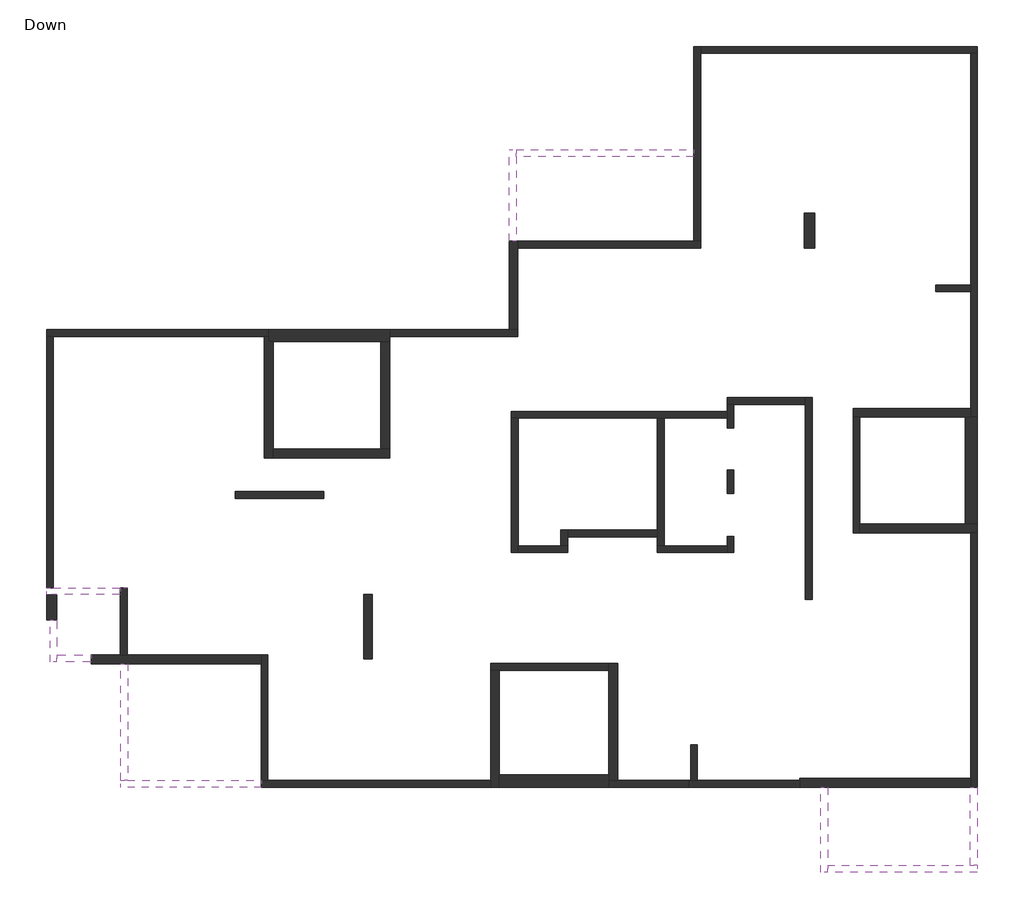
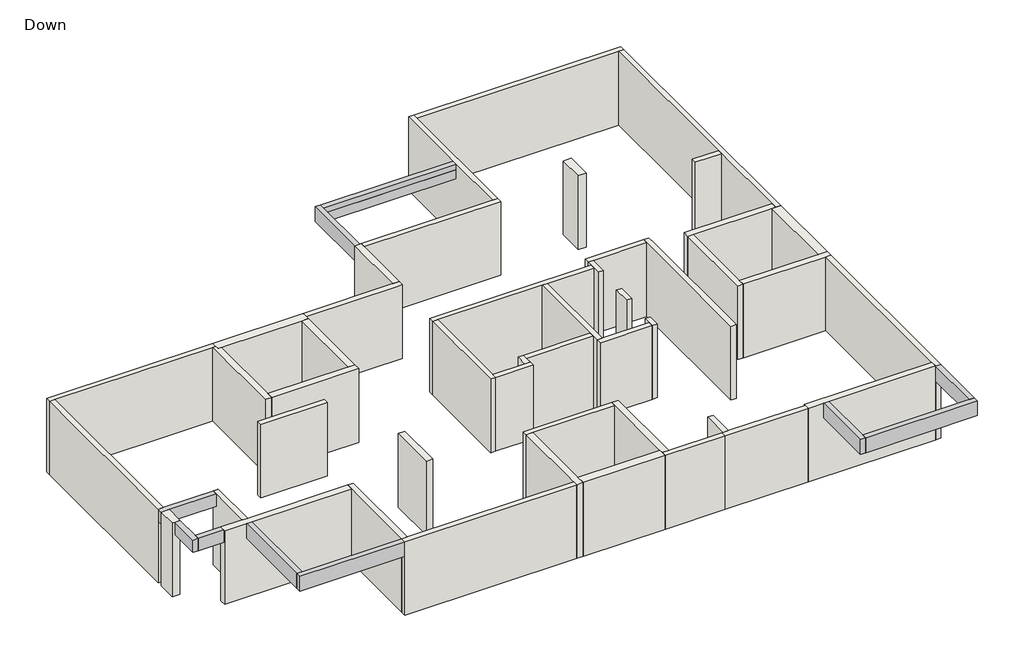
# One storey: 46 walls, 10 beams.
"""IFC4 building model written with IfcOpenShell, lengths in millimetres."""

from ifc_helpers import new_model, si_unit, frame, origin, place, context, project, spatial, polyline, outline, extrude, faceted_brep, element, save

model = new_model("IFC4")

# Units and contexts
model_context = context("Model", 3, world=origin())
ifc_project = project(units=[si_unit("LENGTHUNIT", "METRE", prefix="MILLI")], contexts=[model_context])

# Site, building, storey
site = spatial("IfcSite", under=ifc_project)
building = spatial("IfcBuilding", under=site)
storey = spatial("IfcBuildingStorey", under=building, Name="Down", Elevation=0.0)

# Beams
placement = place(None, origin())
element("IfcBeam", 1, ObjectType="Concrete Rectengular Beam : 20/50", at=placement, inside=storey, context=model_context, shape_type="Brep", body=[
    faceted_brep([(-17264.6329455, 698.5534768, 3000.0), (-17264.6329455, 502.021863, 3000.0), (-16964.6329455, 502.021863, 3000.0), (-15146.7835264, 502.021863, 3000.0), (-15146.7835264, 701.4062462, 3000.0), (-14946.7835264, 701.4062462, 3000.0), (-14946.7835264, 702.021863, 3000.0), (-17064.6329455, 702.021863, 3000.0), (-17064.6329455, 698.5534768, 3000.0), (-17264.6329455, 502.021863, 2500.0), (-15146.7835264, 502.021863, 2500.0), (-15146.7835264, 502.021863, 2770.0), (-17264.6329455, 698.5534768, 2500.0), (-17064.6329455, 698.5534768, 2500.0), (-17064.6329455, 702.021863, 2500.0), (-14946.7835264, 702.021863, 2500.0), (-14946.7835264, 701.4062462, 2500.0), (-15146.7835264, 701.4062462, 2500.0), (-14946.7835264, 702.021863, 2770.0), (-17064.6329455, 702.021863, 2770.0), (-14946.7835264, 701.4062462, 2770.0)], [[[0, 1, 2, 3, 4, 5, 6, 7, 8]], [[1, 9, 10, 11, 3, 2]], [[9, 12, 13, 14, 15, 16, 17, 10]], [[7, 6, 18, 15, 14, 19]], [[9, 1, 0, 12]], [[13, 8, 7, 19, 14]], [[8, 13, 12, 0]], [[17, 4, 3, 11, 10]], [[4, 17, 16, 20, 5]], [[6, 5, 20, 16, 15, 18]]]),
])
element("IfcBeam", 2, ObjectType="Concrete Rectengular Beam : 20/50", at=placement, inside=storey, context=model_context, shape_type="Brep", body=[
    faceted_brep([(-16964.6329455, -228.1954104, 3000.0), (-17164.6329455, -228.1954104, 3000.0), (-17164.6329455, -1438.4211868, 3000.0), (-16964.6329455, -1438.4211868, 3000.0), (-16964.6329455, -1238.4211868, 3000.0), (-17164.6329455, -228.1954104, 2500.0), (-17164.6329455, -1438.4211868, 2500.0), (-16964.6329455, -228.1954104, 2500.0), (-16964.6329455, -1238.4211868, 2500.0), (-16964.6329455, -1438.4211868, 2500.0)], [[[0, 1, 2, 3, 4]], [[1, 5, 6, 2]], [[5, 7, 8, 9, 6]], [[7, 0, 4, 3, 9, 8]], [[1, 0, 7, 5]], [[3, 2, 6, 9]]]),
])
element("IfcBeam", 3, ObjectType="Concrete Rectengular Beam : 20/50", at=placement, inside=storey, context=model_context, shape_type="Brep", body=[
    faceted_brep([(-16964.6329455, -1238.4211868, 3000.0), (-16964.6329455, -1438.4211868, 3000.0), (-15973.5725457, -1438.4211868, 3000.0), (-15973.5725457, -1238.4211868, 3000.0), (-16964.6329455, -1438.4211868, 2500.0), (-15973.5725457, -1438.4211868, 2500.0), (-16964.6329455, -1238.4211868, 2500.0), (-15973.5725457, -1238.4211868, 2500.0), (-16964.6329455, -1238.4211868, 2770.0)], [[[0, 1, 2, 3]], [[1, 4, 5, 2]], [[4, 6, 7, 5]], [[6, 8, 0, 3, 7]], [[1, 0, 8, 6, 4]], [[3, 2, 5, 7]]]),
])
element("IfcBeam", 4, ObjectType="Concrete Rectengular Beam : 20/60", at=placement, inside=storey, context=model_context, shape_type="Brep", body=[
    faceted_brep([(5007.3280344, -7493.4211868, 3000.0), (5207.3280344, -7493.4211868, 3000.0), (5207.3280344, -7293.4211868, 3000.0), (5207.3280344, -5038.4211868, 3000.0), (5007.3280344, -5038.4211868, 3000.0), (5007.3280344, -7493.4211868, 2400.0), (5007.3280344, -5038.4211868, 2400.0), (5207.3280344, -7493.4211868, 2400.0), (5207.3280344, -5038.4211868, 2400.0), (5207.3280344, -7293.4211868, 2400.0), (5207.3280344, -5038.4211868, 2770.0)], [[[0, 1, 2, 3, 4]], [[5, 0, 4, 6]], [[7, 5, 6, 8, 9]], [[1, 7, 9, 8, 10, 3, 2]], [[4, 3, 10, 8, 6]], [[1, 0, 5, 7]]]),
])
element("IfcBeam", 5, ObjectType="Concrete Rectengular Beam : 20/60", at=placement, inside=storey, context=model_context, shape_type="Brep", body=[
    faceted_brep([(9507.3280344, -7493.4211868, 3000.0), (9507.3280344, -7293.4211868, 3000.0), (9307.3280344, -7293.4211868, 3000.0), (5207.3280344, -7293.4211868, 3000.0), (5207.3280344, -7493.4211868, 3000.0), (9507.3280344, -7493.4211868, 2400.0), (5207.3280344, -7493.4211868, 2400.0), (9507.3280344, -7293.4211868, 2400.0), (5207.3280344, -7293.4211868, 2400.0), (9307.3280344, -7293.4211868, 2400.0), (5207.3280344, -7293.4211868, 2770.0)], [[[0, 1, 2, 3, 4]], [[5, 0, 4, 6]], [[7, 5, 6, 8, 9]], [[1, 7, 9, 8, 10, 3, 2]], [[4, 3, 10, 8, 6]], [[1, 0, 5, 7]]]),
])
element("IfcBeam", 6, ObjectType="Concrete Rectengular Beam : 20/60", at=placement, inside=storey, context=model_context, shape_type="Brep", body=[
    faceted_brep([(9507.3280344, -5038.4211868, 3000.0), (9316.8868152, -5038.4211868, 3000.0), (9307.3280344, -5038.4211868, 3000.0), (9307.3280344, -7293.4211868, 3000.0), (9507.3280344, -7293.4211868, 3000.0), (9507.3280344, -7293.4211868, 2400.0), (9507.3280344, -5038.4211868, 2400.0), (9307.3280344, -5038.4211868, 2400.0), (9307.3280344, -7293.4211868, 2400.0), (9307.3280344, -5038.4211868, 2770.0), (9307.3280344, -7293.4211868, 2770.0)], [[[0, 1, 2, 3, 4]], [[4, 5, 6, 0]], [[7, 6, 5, 8]], [[2, 9, 7, 8, 10, 3]], [[0, 6, 7, 9, 2, 1]], [[4, 3, 10, 8, 5]]]),
])
element("IfcBeam", 7, ObjectType="Concrete Rectengular Beam : 20/60", at=placement, inside=storey, context=model_context, shape_type="Brep", body=[
    faceted_brep([(-15133.5932474, -4838.4211868, 3000.0), (-15133.5932474, -5038.4211868, 3000.0), (-11093.5932474, -5038.4211868, 3000.0), (-11093.5932474, -4838.4211868, 3000.0), (-14933.5932474, -4838.4211868, 3000.0), (-15133.5932474, -4838.4211868, 2400.0), (-11093.5932474, -4838.4211868, 2770.0), (-11093.5932474, -4838.4211868, 2400.0), (-14933.5932474, -4838.4211868, 2400.0), (-15133.5932474, -5038.4211868, 2400.0), (-11093.5932474, -5038.4211868, 2400.0)], [[[0, 1, 2, 3, 4]], [[5, 0, 4, 3, 6, 7, 8]], [[9, 5, 8, 7, 10]], [[1, 9, 10, 2]], [[3, 2, 10, 7, 6]], [[1, 0, 5, 9]]]),
])
element("IfcBeam", 8, ObjectType="Concrete Rectengular Beam : 20/60", at=placement, inside=storey, context=model_context, shape_type="Brep", body=[
    faceted_brep([(-14933.5932474, -1488.4211868, 3000.0), (-15133.5932474, -1488.4211868, 3000.0), (-15133.5932474, -4838.4211868, 3000.0), (-14933.5932474, -4838.4211868, 3000.0), (-14933.5932474, -1488.4211868, 2400.0), (-14933.5932474, -1488.4211868, 2770.0), (-14933.5932474, -4838.4211868, 2770.0), (-14933.5932474, -4838.4211868, 2400.0), (-15133.5932474, -1488.4211868, 2400.0), (-15133.5932474, -4838.4211868, 2400.0)], [[[0, 1, 2, 3]], [[4, 5, 0, 3, 6, 7]], [[8, 4, 7, 9]], [[1, 8, 9, 2]], [[1, 0, 5, 4, 8]], [[3, 2, 9, 7, 6]]]),
])
element("IfcBeam", 9, ObjectType="Concrete Rectengular Beam : 20/60", at=placement, inside=storey, context=model_context, shape_type="Brep", body=[
    faceted_brep([(-3753.1131848, 13310.0948632, 3000.0), (-3953.1131848, 13310.0948632, 3000.0), (-3953.1131848, 10680.6924355, 3000.0), (-3754.7272111, 10680.6924355, 3000.0), (-3754.7272111, 13112.8657791, 3000.0), (-3753.1131848, 13112.8657791, 3000.0), (-3753.1131848, 13310.0948632, 2400.0), (-3753.1131848, 13112.8657791, 2770.0), (-3753.1131848, 13110.0948632, 2770.0), (-3753.1131848, 10680.6924355, 2770.0), (-3753.1131848, 10680.6924355, 2400.0), (-3753.1131848, 13110.0948632, 2400.0), (-3953.1131848, 10680.6924355, 2400.0), (-3953.1131848, 13310.0948632, 2400.0), (-3754.7272111, 10680.6924355, 2770.0), (-3754.7272111, 13112.8657791, 2770.0)], [[[0, 1, 2, 3, 4, 5]], [[6, 0, 5, 7, 8, 9, 10, 11]], [[10, 12, 13, 6, 11]], [[12, 2, 1, 13]], [[12, 10, 9, 14, 3, 2]], [[1, 0, 6, 13]], [[15, 14, 9, 8, 7]], [[14, 15, 4, 3]], [[4, 15, 7, 5]]]),
])
element("IfcBeam", 10, ObjectType="Concrete Rectengular Beam : 20/60", at=placement, inside=storey, context=model_context, shape_type="SweptSolid", body=[
    extrude(outline(polyline([(13310.0948632, 2400.0), (13110.0948632, 2400.0), (13110.0948632, 2770.0), (13112.8657791, 2770.0), (13112.8657791, 3000.0), (13310.0948632, 3000.0), (13310.0948632, 2400.0)])), frame((-3753.1131848, 0.0, 0.0), z_axis=(1.0, 0.0, 0.0), x_axis=(0.0, 1.0, 0.0)), (0.0, 0.0, 1.0), 5110.0),
])

# Walls
element("IfcWall", 11, ObjectType="20", at=placement, inside=storey, context=model_context, shape_type="Brep", body=[
    faceted_brep([(-17264.6329455, 7938.5534768, 0.0), (-17064.6329455, 7938.5534768, 0.0), (-10996.4058847, 7938.5534768, 0.0), (-10871.4058847, 7938.5534768, 0.0), (-10871.4058847, 7938.5534768, 3000.0), (-10996.4058847, 7938.5534768, 3000.0), (-17064.6329455, 7938.5534768, 3000.0), (-17264.6329455, 7938.5534768, 3000.0), (-17264.6329455, 8138.5534768, 0.0), (-17264.6329455, 8138.5534768, 3000.0), (-10871.4058847, 8138.5534768, 3000.0), (-10871.4058847, 8138.5534768, 0.0)], [[[0, 1, 2, 3, 4, 5, 6, 7]], [[8, 9, 10, 11]], [[3, 2, 1, 0, 8, 11]], [[4, 3, 11, 10]], [[7, 6, 5, 4, 10, 9]], [[0, 7, 9, 8]]]),
])
element("IfcWall", 12, ObjectType="20", at=placement, inside=storey, context=model_context, shape_type="Brep", body=[
    faceted_brep([(-17264.6329455, 7938.5534768, 0.0), (-17264.6329455, 698.5534768, 0.0), (-17264.6329455, 698.5534768, 3000.0), (-17264.6329455, 7938.5534768, 3000.0), (-17064.6329455, 7938.5534768, 0.0), (-17064.6329455, 7938.5534768, 2770.0), (-17064.6329455, 7938.5534768, 3000.0), (-17064.6329455, 702.021863, 3000.0), (-17064.6329455, 698.5534768, 3000.0), (-17064.6329455, 698.5534768, 0.0)], [[[0, 1, 2, 3]], [[4, 5, 6, 7, 8, 9]], [[1, 0, 4, 9]], [[2, 1, 9, 8]], [[3, 2, 8, 7, 6]], [[0, 3, 6, 5, 4]]]),
])
element("IfcWall", 13, ObjectType="20", at=placement, inside=storey, context=model_context, shape_type="Brep", body=[
    faceted_brep([(-7397.5153815, 7938.5534768, 0.0), (-3703.1131848, 7938.5534768, 0.0), (-3703.1131848, 7938.5534768, 2770.0), (-3703.1131848, 7938.5534768, 3000.0), (-3898.2455034, 7938.5534768, 3000.0), (-7397.5153815, 7938.5534768, 3000.0), (-7397.5153815, 7938.5534768, 2770.0), (-7397.5153815, 8138.5534768, 0.0), (-7397.5153815, 8138.5534768, 3000.0), (-3953.1131848, 8138.5534768, 3000.0), (-3703.1131848, 8138.5534768, 3000.0), (-3703.1131848, 8138.5534768, 0.0), (-3953.1131848, 8138.5534768, 0.0)], [[[0, 1, 2, 3, 4, 5, 6]], [[7, 8, 9, 10, 11, 12]], [[1, 0, 7, 12, 11]], [[5, 4, 3, 10, 9, 8]], [[0, 6, 5, 8, 7]], [[3, 2, 1, 11, 10]]]),
])
element("IfcWall", 14, ObjectType="20", at=placement, inside=storey, context=model_context, shape_type="Brep", body=[
    faceted_brep([(-3703.1131848, 10480.6924355, 0.0), (1556.8868152, 10480.6924355, 0.0), (1556.8868152, 10480.6924355, 2770.0), (1556.8868152, 10480.6924355, 3000.0), (-3703.1131848, 10480.6924355, 3000.0), (-3703.1131848, 10480.6924355, 2770.0), (-3703.1131848, 10680.6924355, 0.0), (-3703.1131848, 10680.6924355, 3000.0), (1356.8868152, 10680.6924355, 3000.0), (1556.8868152, 10680.6924355, 3000.0), (1556.8868152, 10680.6924355, 0.0), (1356.8868152, 10680.6924355, 0.0)], [[[0, 1, 2, 3, 4, 5]], [[6, 7, 8, 9, 10, 11]], [[1, 0, 6, 11, 10]], [[4, 3, 9, 8, 7]], [[0, 5, 4, 7, 6]], [[3, 2, 1, 10, 9]]]),
])
element("IfcWall", 15, ObjectType="20", at=placement, inside=storey, context=model_context, shape_type="Brep", body=[
    faceted_brep([(1556.8868152, 10680.6924355, 0.0), (1556.8868152, 16080.6924355, 0.0), (1556.8868152, 16280.6924355, 0.0), (1556.8868152, 16280.6924355, 3000.0), (1556.8868152, 16080.6924355, 3000.0), (1556.8868152, 10680.6924355, 3000.0), (1356.8868152, 10680.6924355, 0.0), (1356.8868152, 10680.6924355, 2770.0), (1356.8868152, 10680.6924355, 3000.0), (1356.8868152, 13112.8657791, 3000.0), (1356.8868152, 16280.6924355, 3000.0), (1356.8868152, 16280.6924355, 0.0)], [[[0, 1, 2, 3, 4, 5]], [[6, 7, 8, 9, 10, 11]], [[2, 1, 0, 6, 11]], [[5, 4, 3, 10, 9, 8]], [[0, 5, 8, 7, 6]], [[3, 2, 11, 10]]]),
])
element("IfcWall", 16, ObjectType="20", at=placement, inside=storey, context=model_context, shape_type="Brep", body=[
    faceted_brep([(1556.8868152, 16080.6924355, 0.0), (9316.8868152, 16080.6924355, 0.0), (9516.8868152, 16080.6924355, 0.0), (9516.8868152, 16080.6924355, 3000.0), (9316.8868152, 16080.6924355, 3000.0), (1556.8868152, 16080.6924355, 3000.0), (1556.8868152, 16080.6924355, 2770.0), (1556.8868152, 16280.6924355, 0.0), (1556.8868152, 16280.6924355, 3000.0), (9516.8868152, 16280.6924355, 3000.0), (9516.8868152, 16280.6924355, 0.0)], [[[0, 1, 2, 3, 4, 5, 6]], [[7, 8, 9, 10]], [[2, 1, 0, 7, 10]], [[5, 4, 3, 9, 8]], [[0, 6, 5, 8, 7]], [[3, 2, 10, 9]]]),
])
element("IfcWall", 17, ObjectType="20", at=placement, inside=storey, context=model_context, shape_type="Brep", body=[
    faceted_brep([(9316.8868152, 16080.6924355, 0.0), (9316.8868152, 9419.5945609, 0.0), (9316.8868152, 9219.5945609, 0.0), (9316.8868152, 5860.6924355, 0.0), (9316.8868152, 5610.6924355, 0.0), (9316.8868152, 5610.6924355, 3000.0), (9316.8868152, 5860.6924355, 3000.0), (9316.8868152, 9219.5945609, 3000.0), (9316.8868152, 9419.5945609, 3000.0), (9316.8868152, 16080.6924355, 3000.0), (9316.8868152, 16080.6924355, 2770.0), (9516.8868152, 16080.6924355, 0.0), (9516.8868152, 16080.6924355, 3000.0), (9516.8868152, 5610.6924355, 3000.0), (9516.8868152, 5610.6924355, 0.0)], [[[0, 1, 2, 3, 4, 5, 6, 7, 8, 9, 10]], [[11, 12, 13, 14]], [[4, 3, 2, 1, 0, 11, 14]], [[9, 8, 7, 6, 5, 13, 12]], [[0, 10, 9, 12, 11]], [[5, 4, 14, 13]]]),
])
element("IfcWall", 18, ObjectType="20", at=placement, inside=storey, context=model_context, shape_type="Brep", body=[
    faceted_brep([(5936.8868152, 5610.6924355, 0.0), (5936.8868152, 2281.5477607, 0.0), (5936.8868152, 2281.5477607, 2770.0), (5936.8868152, 2281.5477607, 3000.0), (5936.8868152, 5610.6924355, 3000.0), (6136.8868152, 5610.6924355, 0.0), (6136.8868152, 5610.6924355, 2770.0), (6136.8868152, 5610.6924355, 3000.0), (6136.8868152, 2531.5477607, 3000.0), (6136.8868152, 2281.5477607, 3000.0), (6136.8868152, 2281.5477607, 0.0), (6136.8868152, 2531.5477607, 0.0)], [[[0, 1, 2, 3, 4]], [[5, 6, 7, 8, 9, 10, 11]], [[1, 0, 5, 11, 10]], [[4, 3, 9, 8, 7]], [[0, 4, 7, 6, 5]], [[3, 2, 1, 10, 9]]]),
])
element("IfcWall", 19, ObjectType="20", at=placement, inside=storey, context=model_context, shape_type="Brep", body=[
    faceted_brep([(9316.8868152, 2281.5477607, 0.0), (9316.8868152, -4788.4211868, 0.0), (9316.8868152, -5038.4211868, 0.0), (9316.8868152, -5038.4211868, 3000.0), (9316.8868152, -4788.4211868, 3000.0), (9316.8868152, 2281.5477607, 3000.0), (9316.8868152, 2281.5477607, 2770.0), (9516.8868152, 2281.5477607, 0.0), (9516.8868152, 2281.5477607, 3000.0), (9516.8868152, -5038.4211868, 3000.0), (9516.8868152, -5038.4211868, 0.0), (9507.3280344, -5038.4211868, 3000.0)], [[[0, 1, 2, 3, 4, 5, 6]], [[7, 8, 9, 10]], [[2, 1, 0, 7, 10]], [[5, 4, 3, 11, 9, 8]], [[0, 6, 5, 8, 7]], [[3, 2, 10, 9, 11]]]),
])
element("IfcWall", 20, ObjectType="20", at=placement, inside=storey, context=model_context, shape_type="Brep", body=[
    faceted_brep([(4411.1547291, -4838.4211868, 0.0), (1462.7563726, -4838.4211868, 0.0), (1262.7563726, -4838.4211868, 0.0), (1210.9852813, -4838.4211868, 0.0), (1210.9852813, -4838.4211868, 3000.0), (1262.7563726, -4838.4211868, 3000.0), (1462.7563726, -4838.4211868, 3000.0), (4411.1547291, -4838.4211868, 3000.0), (4411.1547291, -4838.4211868, 2770.0), (4411.1547291, -5038.4211868, 0.0), (4411.1547291, -5038.4211868, 3000.0), (1210.9852813, -5038.4211868, 3000.0), (1210.9852813, -5038.4211868, 0.0)], [[[0, 1, 2, 3, 4, 5, 6, 7, 8]], [[9, 10, 11, 12]], [[3, 2, 1, 0, 9, 12]], [[4, 3, 12, 11]], [[7, 6, 5, 4, 11, 10]], [[0, 8, 7, 10, 9]]]),
])
element("IfcWall", 21, ObjectType="20", at=placement, inside=storey, context=model_context, shape_type="Brep", body=[
    faceted_brep([(1462.7563726, -4838.4211868, 0.0), (1462.7563726, -3819.6429934, 0.0), (1462.7563726, -3819.6429934, 2770.0), (1462.7563726, -3819.6429934, 3000.0), (1462.7563726, -4838.4211868, 3000.0), (1462.7563726, -4838.4211868, 2770.0), (1262.7563726, -4838.4211868, 0.0), (1262.7563726, -4838.4211868, 2770.0), (1262.7563726, -4838.4211868, 3000.0), (1262.7563726, -3819.6429934, 3000.0), (1262.7563726, -3819.6429934, 2770.0), (1262.7563726, -3819.6429934, 0.0)], [[[0, 1, 2, 3, 4, 5]], [[6, 7, 8, 9, 10, 11]], [[1, 0, 6, 11]], [[3, 2, 1, 11, 10, 9]], [[4, 3, 9, 8]], [[0, 5, 4, 8, 7, 6]]]),
])
element("IfcWall", 22, ObjectType="20", at=placement, inside=storey, context=model_context, shape_type="Brep", body=[
    faceted_brep([(1210.9852813, -4838.4211868, 0.0), (-837.6785216, -4838.4211868, 0.0), (-1087.6785216, -4838.4211868, 0.0), (-1087.6785216, -4838.4211868, 3000.0), (-837.6785216, -4838.4211868, 3000.0), (1210.9852813, -4838.4211868, 3000.0), (1210.9852813, -5038.4211868, 0.0), (1210.9852813, -5038.4211868, 3000.0), (-1087.6785216, -5038.4211868, 3000.0), (-1087.6785216, -5038.4211868, 0.0)], [[[0, 1, 2, 3, 4, 5]], [[6, 7, 8, 9]], [[2, 1, 0, 6, 9]], [[5, 4, 3, 8, 7]], [[0, 5, 7, 6]], [[3, 2, 9, 8]]]),
])
element("IfcWall", 23, ObjectType="20", at=placement, inside=storey, context=model_context, shape_type="Brep", body=[
    faceted_brep([(-1087.6785216, -1479.3693914, 0.0), (-4486.4747594, -1479.3693914, 0.0), (-4486.4747594, -1479.3693914, 2770.0), (-4486.4747594, -1479.3693914, 3000.0), (-1087.6785216, -1479.3693914, 3000.0), (-1087.6785216, -1679.3693914, 0.0), (-1087.6785216, -1679.3693914, 2770.0), (-1087.6785216, -1679.3693914, 3000.0), (-4236.4747594, -1679.3693914, 3000.0), (-4486.4747594, -1679.3693914, 3000.0), (-4486.4747594, -1679.3693914, 0.0), (-4236.4747594, -1679.3693914, 0.0)], [[[0, 1, 2, 3, 4]], [[5, 6, 7, 8, 9, 10, 11]], [[1, 0, 5, 11, 10]], [[4, 3, 9, 8, 7]], [[0, 4, 7, 6, 5]], [[3, 2, 1, 10, 9]]]),
])
element("IfcWall", 24, ObjectType="20", at=placement, inside=storey, context=model_context, shape_type="Brep", body=[
    faceted_brep([(-4486.4747594, -4838.4211868, 0.0), (-10893.5932474, -4838.4211868, 0.0), (-11093.5932474, -4838.4211868, 0.0), (-11093.5932474, -4838.4211868, 2400.0), (-11093.5932474, -4838.4211868, 3000.0), (-10893.5932474, -4838.4211868, 3000.0), (-4486.4747594, -4838.4211868, 3000.0), (-4486.4747594, -4838.4211868, 2770.0), (-4486.4747594, -5038.4211868, 0.0), (-4486.4747594, -5038.4211868, 3000.0), (-11093.5932474, -5038.4211868, 3000.0), (-11093.5932474, -5038.4211868, 2400.0), (-11093.5932474, -5038.4211868, 0.0)], [[[0, 1, 2, 3, 4, 5, 6, 7]], [[8, 9, 10, 11, 12]], [[2, 1, 0, 8, 12]], [[6, 5, 4, 10, 9]], [[0, 7, 6, 9, 8]], [[4, 3, 2, 12, 11, 10]]]),
])
element("IfcWall", 25, ObjectType="20", at=placement, inside=storey, context=model_context, shape_type="Brep", body=[
    faceted_brep([(-10893.5932474, -4838.4211868, 0.0), (-10893.5932474, -1238.4211868, 0.0), (-10893.5932474, -1238.4211868, 2770.0), (-10893.5932474, -1238.4211868, 3000.0), (-10893.5932474, -4838.4211868, 3000.0), (-10893.5932474, -4838.4211868, 2770.0), (-11093.5932474, -4838.4211868, 0.0), (-11093.5932474, -4838.4211868, 2770.0), (-11093.5932474, -4838.4211868, 3000.0), (-11093.5932474, -1488.4211868, 3000.0), (-11093.5932474, -1238.4211868, 3000.0), (-11093.5932474, -1238.4211868, 0.0), (-11093.5932474, -1488.4211868, 0.0)], [[[0, 1, 2, 3, 4, 5]], [[6, 7, 8, 9, 10, 11, 12]], [[1, 0, 6, 12, 11]], [[4, 3, 10, 9, 8]], [[0, 5, 4, 8, 7, 6]], [[3, 2, 1, 11, 10]]]),
])
element("IfcWall", 26, ObjectType="20", at=placement, inside=storey, context=model_context, shape_type="Brep", body=[
    faceted_brep([(-14946.7835264, -1238.4211868, 0.0), (-14946.7835264, 701.4062462, 0.0), (-14946.7835264, 701.4062462, 2500.0), (-14946.7835264, 701.4062462, 3000.0), (-14946.7835264, -1238.4211868, 3000.0), (-14946.7835264, -1238.4211868, 2770.0), (-15146.7835264, -1238.4211868, 0.0), (-15146.7835264, -1238.4211868, 2770.0), (-15146.7835264, -1238.4211868, 3000.0), (-15146.7835264, 502.021863, 3000.0), (-15146.7835264, 701.4062462, 3000.0), (-15146.7835264, 701.4062462, 2500.0), (-15146.7835264, 701.4062462, 0.0)], [[[0, 1, 2, 3, 4, 5]], [[6, 7, 8, 9, 10, 11, 12]], [[1, 0, 6, 12]], [[3, 2, 1, 12, 11, 10]], [[4, 3, 10, 9, 8]], [[0, 5, 4, 8, 7, 6]]]),
])
element("IfcWall", 27, ObjectType="20", at=placement, inside=storey, context=model_context, shape_type="Brep", body=[
    faceted_brep([(9316.8868152, 9419.5945609, 0.0), (8313.9644764, 9419.5945609, 0.0), (8313.9644764, 9419.5945609, 2770.0), (8313.9644764, 9419.5945609, 3000.0), (9316.8868152, 9419.5945609, 3000.0), (9316.8868152, 9419.5945609, 2770.0), (9316.8868152, 9219.5945609, 0.0), (9316.8868152, 9219.5945609, 2770.0), (9316.8868152, 9219.5945609, 3000.0), (8313.9644764, 9219.5945609, 3000.0), (8313.9644764, 9219.5945609, 2770.0), (8313.9644764, 9219.5945609, 0.0)], [[[0, 1, 2, 3, 4, 5]], [[6, 7, 8, 9, 10, 11]], [[1, 0, 6, 11]], [[3, 2, 1, 11, 10, 9]], [[4, 3, 9, 8]], [[0, 5, 4, 8, 7, 6]]]),
])
element("IfcWall", 28, ObjectType="20", at=placement, inside=storey, context=model_context, shape_type="Brep", body=[
    faceted_brep([(-9286.68122, 3466.0170988, 0.0), (-11831.3488632, 3466.0170988, 0.0), (-11831.3488632, 3466.0170988, 2770.0), (-11831.3488632, 3466.0170988, 3000.0), (-9286.68122, 3466.0170988, 3000.0), (-9286.68122, 3466.0170988, 2770.0), (-9286.68122, 3266.0170988, 0.0), (-9286.68122, 3266.0170988, 2770.0), (-9286.68122, 3266.0170988, 3000.0), (-11831.3488632, 3266.0170988, 3000.0), (-11831.3488632, 3266.0170988, 2770.0), (-11831.3488632, 3266.0170988, 0.0)], [[[0, 1, 2, 3, 4, 5]], [[6, 7, 8, 9, 10, 11]], [[1, 0, 6, 11]], [[3, 2, 1, 11, 10, 9]], [[4, 3, 9, 8]], [[0, 5, 4, 8, 7, 6]]]),
])
element("IfcWall", 29, ObjectType="20", at=placement, inside=storey, context=model_context, shape_type="Brep", body=[
    faceted_brep([(4760.6810887, 359.9861346, 0.0), (4760.6810887, 6179.5864053, 0.0), (4760.6810887, 6179.5864053, 2770.0), (4760.6810887, 6179.5864053, 3000.0), (4760.6810887, 5860.6924355, 3000.0), (4760.6810887, 359.9861346, 3000.0), (4760.6810887, 359.9861346, 2770.0), (4560.6810887, 359.9861346, 0.0), (4560.6810887, 359.9861346, 2770.0), (4560.6810887, 359.9861346, 3000.0), (4560.6810887, 1710.8284517, 3000.0), (4560.6810887, 5979.5864053, 3000.0), (4560.6810887, 6179.5864053, 3000.0), (4560.6810887, 6179.5864053, 0.0), (4560.6810887, 5979.5864053, 0.0)], [[[0, 1, 2, 3, 4, 5, 6]], [[7, 8, 9, 10, 11, 12, 13, 14]], [[1, 0, 7, 14, 13]], [[5, 4, 3, 12, 11, 10, 9]], [[0, 6, 5, 9, 8, 7]], [[3, 2, 1, 13, 12]]]),
])
element("IfcWall", 30, ObjectType="20", at=placement, inside=storey, context=model_context, shape_type="Brep", body=[
    faceted_brep([(4560.6810887, 6179.5864053, 0.0), (2312.6329026, 6179.5864053, 0.0), (2312.6329026, 6179.5864053, 2770.0), (2312.6329026, 6179.5864053, 3000.0), (4560.6810887, 6179.5864053, 3000.0), (4560.6810887, 5979.5864053, 0.0), (4560.6810887, 5979.5864053, 2770.0), (4560.6810887, 5979.5864053, 3000.0), (2512.6329026, 5979.5864053, 3000.0), (2312.6329026, 5979.5864053, 3000.0), (2312.6329026, 5979.5864053, 0.0), (2512.6329026, 5979.5864053, 0.0)], [[[0, 1, 2, 3, 4]], [[5, 6, 7, 8, 9, 10, 11]], [[1, 0, 5, 11, 10]], [[4, 3, 9, 8, 7]], [[0, 4, 7, 6, 5]], [[3, 2, 1, 10, 9]]]),
])
element("IfcWall", 31, ObjectType="20", at=placement, inside=storey, context=model_context, shape_type="Brep", body=[
    faceted_brep([(2312.6329026, 5979.5864053, 0.0), (2312.6329026, 5780.7699278, 0.0), (2312.6329026, 5580.7699278, 0.0), (2312.6329026, 5304.757008, 0.0), (2312.6329026, 5304.757008, 2770.0), (2312.6329026, 5304.757008, 3000.0), (2312.6329026, 5580.7699278, 3000.0), (2312.6329026, 5780.7699278, 3000.0), (2312.6329026, 5979.5864053, 3000.0), (2512.6329026, 5979.5864053, 0.0), (2512.6329026, 5979.5864053, 2770.0), (2512.6329026, 5979.5864053, 3000.0), (2512.6329026, 5304.757008, 3000.0), (2512.6329026, 5304.757008, 2770.0), (2512.6329026, 5304.757008, 0.0)], [[[0, 1, 2, 3, 4, 5, 6, 7, 8]], [[9, 10, 11, 12, 13, 14]], [[3, 2, 1, 0, 9, 14]], [[5, 4, 3, 14, 13, 12]], [[8, 7, 6, 5, 12, 11]], [[0, 8, 11, 10, 9]]]),
])
element("IfcWall", 32, ObjectType="20", at=placement, inside=storey, context=model_context, shape_type="Brep", body=[
    faceted_brep([(2312.6329026, 5780.7699278, 0.0), (-3898.2455034, 5780.7699278, 0.0), (-3898.2455034, 5780.7699278, 2770.0), (-3898.2455034, 5780.7699278, 3000.0), (2312.6329026, 5780.7699278, 3000.0), (2312.6329026, 5780.7699278, 2770.0), (2312.6329026, 5580.7699278, 0.0), (2312.6329026, 5580.7699278, 3000.0), (511.2984388, 5580.7699278, 3000.0), (311.2984388, 5580.7699278, 3000.0), (-3698.2455034, 5580.7699278, 3000.0), (-3898.2455034, 5580.7699278, 3000.0), (-3898.2455034, 5580.7699278, 0.0), (-3698.2455034, 5580.7699278, 0.0), (311.2984388, 5580.7699278, 0.0), (511.2984388, 5580.7699278, 0.0)], [[[0, 1, 2, 3, 4, 5]], [[6, 7, 8, 9, 10, 11, 12, 13, 14, 15]], [[1, 0, 6, 15, 14, 13, 12]], [[4, 3, 11, 10, 9, 8, 7]], [[0, 5, 4, 7, 6]], [[3, 2, 1, 12, 11]]]),
])
element("IfcWall", 33, ObjectType="20", at=placement, inside=storey, context=model_context, shape_type="Brep", body=[
    faceted_brep([(-3898.2455034, 5580.7699278, 0.0), (-3898.2455034, 1710.8284517, 0.0), (-3898.2455034, 1710.8284517, 2770.0), (-3898.2455034, 1710.8284517, 3000.0), (-3898.2455034, 5580.7699278, 3000.0), (-3698.2455034, 5580.7699278, 0.0), (-3698.2455034, 5580.7699278, 3000.0), (-3698.2455034, 1910.8284517, 3000.0), (-3698.2455034, 1710.8284517, 3000.0), (-3698.2455034, 1710.8284517, 0.0), (-3698.2455034, 1910.8284517, 0.0)], [[[0, 1, 2, 3, 4]], [[5, 6, 7, 8, 9, 10]], [[1, 0, 5, 10, 9]], [[4, 3, 8, 7, 6]], [[0, 4, 6, 5]], [[3, 2, 1, 9, 8]]]),
])
element("IfcWall", 34, ObjectType="20", at=placement, inside=storey, context=model_context, shape_type="Brep", body=[
    faceted_brep([(-3698.2455034, 1710.8284517, 0.0), (-2268.2936764, 1710.8284517, 0.0), (-2268.2936764, 1710.8284517, 2770.0), (-2268.2936764, 1710.8284517, 3000.0), (-3698.2455034, 1710.8284517, 3000.0), (-3698.2455034, 1910.8284517, 0.0), (-3698.2455034, 1910.8284517, 3000.0), (-2468.2936764, 1910.8284517, 3000.0), (-2268.2936764, 1910.8284517, 3000.0), (-2268.2936764, 1910.8284517, 0.0), (-2468.2936764, 1910.8284517, 0.0)], [[[0, 1, 2, 3, 4]], [[5, 6, 7, 8, 9, 10]], [[1, 0, 5, 10, 9]], [[4, 3, 8, 7, 6]], [[0, 4, 6, 5]], [[3, 2, 1, 9, 8]]]),
])
element("IfcWall", 35, ObjectType="20", at=placement, inside=storey, context=model_context, shape_type="Brep", body=[
    faceted_brep([(-2268.2936764, 1910.8284517, 0.0), (-2268.2936764, 2161.3205984, 0.0), (-2268.2936764, 2361.3205984, 0.0), (-2268.2936764, 2361.3205984, 3000.0), (-2268.2936764, 2161.3205984, 3000.0), (-2268.2936764, 1910.8284517, 3000.0), (-2468.2936764, 1910.8284517, 0.0), (-2468.2936764, 1910.8284517, 3000.0), (-2468.2936764, 2361.3205984, 3000.0), (-2468.2936764, 2361.3205984, 0.0)], [[[0, 1, 2, 3, 4, 5]], [[6, 7, 8, 9]], [[2, 1, 0, 6, 9]], [[5, 4, 3, 8, 7]], [[0, 5, 7, 6]], [[3, 2, 9, 8]]]),
])
element("IfcWall", 36, ObjectType="20", at=placement, inside=storey, context=model_context, shape_type="Brep", body=[
    faceted_brep([(-2268.2936764, 2161.3205984, 0.0), (311.2984388, 2161.3205984, 0.0), (311.2984388, 2161.3205984, 2770.0), (311.2984388, 2161.3205984, 3000.0), (-2268.2936764, 2161.3205984, 3000.0), (-2268.2936764, 2161.3205984, 2770.0), (-2268.2936764, 2361.3205984, 0.0), (-2268.2936764, 2361.3205984, 3000.0), (311.2984388, 2361.3205984, 3000.0), (311.2984388, 2361.3205984, 0.0)], [[[0, 1, 2, 3, 4, 5]], [[6, 7, 8, 9]], [[1, 0, 6, 9]], [[4, 3, 8, 7]], [[0, 5, 4, 7, 6]], [[3, 2, 1, 9, 8]]]),
])
element("IfcWall", 37, ObjectType="20", at=placement, inside=storey, context=model_context, shape_type="Brep", body=[
    faceted_brep([(311.2984388, 1710.8284517, 0.0), (2312.0172858, 1710.8284517, 0.0), (2312.0172858, 1710.8284517, 3000.0), (311.2984388, 1710.8284517, 3000.0), (311.2984388, 1710.8284517, 2770.0), (311.2984388, 1910.8284517, 0.0), (311.2984388, 1910.8284517, 3000.0), (511.2984388, 1910.8284517, 3000.0), (2312.0172858, 1910.8284517, 3000.0), (2312.0172858, 1910.8284517, 0.0), (511.2984388, 1910.8284517, 0.0)], [[[0, 1, 2, 3, 4]], [[5, 6, 7, 8, 9, 10]], [[1, 0, 5, 10, 9]], [[3, 2, 8, 7, 6]], [[2, 1, 9, 8]], [[0, 4, 3, 6, 5]]]),
])
element("IfcWall", 38, ObjectType="20", at=placement, inside=storey, context=model_context, shape_type="Brep", body=[
    faceted_brep([(2512.0172858, 1710.8284517, 0.0), (2512.0172858, 2179.3507401, 0.0), (2512.0172858, 2179.3507401, 2770.0), (2512.0172858, 2179.3507401, 3000.0), (2512.0172858, 1710.8284517, 3000.0), (2512.0172858, 1710.8284517, 2770.0), (2312.0172858, 1710.8284517, 0.0), (2312.0172858, 1710.8284517, 3000.0), (2312.0172858, 1910.8284517, 3000.0), (2312.0172858, 2179.3507401, 3000.0), (2312.0172858, 2179.3507401, 0.0), (2312.0172858, 1910.8284517, 0.0), (2312.6329026, 2179.3507401, 3000.0)], [[[0, 1, 2, 3, 4, 5]], [[6, 7, 8, 9, 10, 11]], [[1, 0, 6, 11, 10]], [[3, 2, 1, 10, 9, 12]], [[4, 3, 12, 9, 8, 7]], [[0, 5, 4, 7, 6]]]),
])
element("IfcWall", 39, ObjectType="20", at=placement, inside=storey, context=model_context, shape_type="Brep", body=[
    faceted_brep([(511.2984388, 1910.8284517, 0.0), (511.2984388, 5580.7699278, 0.0), (511.2984388, 5580.7699278, 3000.0), (511.2984388, 1910.8284517, 3000.0), (311.2984388, 1910.8284517, 0.0), (311.2984388, 1910.8284517, 3000.0), (311.2984388, 2161.3205984, 3000.0), (311.2984388, 2361.3205984, 3000.0), (311.2984388, 5580.7699278, 3000.0), (311.2984388, 5580.7699278, 0.0), (311.2984388, 2361.3205984, 0.0), (311.2984388, 2161.3205984, 0.0)], [[[0, 1, 2, 3]], [[4, 5, 6, 7, 8, 9, 10, 11]], [[1, 0, 4, 11, 10, 9]], [[3, 2, 8, 7, 6, 5]], [[2, 1, 9, 8]], [[0, 3, 5, 4]]]),
])
element("IfcWall", 40, ObjectType="20", at=placement, inside=storey, context=model_context, shape_type="Brep", body=[
    faceted_brep([(2512.0172858, 3415.5911695, 0.0), (2512.0172858, 4085.9788147, 0.0), (2512.0172858, 4085.9788147, 2770.0), (2512.0172858, 4085.9788147, 3000.0), (2512.0172858, 3415.5911695, 3000.0), (2512.0172858, 3415.5911695, 2770.0), (2312.0172858, 3415.5911695, 0.0), (2312.0172858, 3415.5911695, 3000.0), (2312.0172858, 4085.9788147, 3000.0), (2312.0172858, 4085.9788147, 0.0), (2312.6329026, 4085.9788147, 3000.0), (2312.6329026, 3415.5911695, 3000.0)], [[[0, 1, 2, 3, 4, 5]], [[6, 7, 8, 9]], [[1, 0, 6, 9]], [[3, 2, 1, 9, 8, 10]], [[4, 3, 10, 8, 7, 11]], [[0, 5, 4, 11, 7, 6]]]),
])
element("IfcWall", 41, ObjectType="25", at=placement, inside=storey, context=model_context, shape_type="Brep", body=[
    faceted_brep([(-10996.4058847, 7938.5534768, 0.0), (-10996.4058847, 4439.8992155, 0.0), (-10996.4058847, 4439.8992155, 2770.0), (-10996.4058847, 4439.8992155, 3000.0), (-10996.4058847, 7938.5534768, 3000.0), (-10996.4058847, 7938.5534768, 2770.0), (-10746.4058847, 7788.5534768, 0.0), (-10746.4058847, 7788.5534768, 2770.0), (-10746.4058847, 7788.5534768, 3000.0), (-10746.4058847, 4689.8992155, 3000.0), (-10746.4058847, 4439.8992155, 3000.0), (-10746.4058847, 4439.8992155, 0.0), (-10746.4058847, 4689.8992155, 0.0), (-10871.4058847, 7938.5534768, 0.0), (-10871.4058847, 7788.5534768, 0.0), (-10871.4058847, 7788.5534768, 3000.0), (-10871.4058847, 7938.5534768, 3000.0)], [[[0, 1, 2, 3, 4, 5]], [[6, 7, 8, 9, 10, 11, 12]], [[1, 0, 13, 14, 6, 12, 11]], [[4, 3, 10, 9, 8, 15, 16]], [[0, 5, 4, 16, 13]], [[16, 15, 14, 13]], [[15, 8, 7, 6, 14]], [[3, 2, 1, 11, 10]]]),
])
element("IfcWall", 42, ObjectType="25", at=placement, inside=storey, context=model_context, shape_type="Brep", body=[
    faceted_brep([(-10746.4058847, 4439.8992155, 0.0), (-7397.5153815, 4439.8992155, 0.0), (-7397.5153815, 4439.8992155, 2770.0), (-7397.5153815, 4439.8992155, 3000.0), (-10746.4058847, 4439.8992155, 3000.0), (-10746.4058847, 4689.8992155, 0.0), (-10746.4058847, 4689.8992155, 2770.0), (-10746.4058847, 4689.8992155, 3000.0), (-7647.5153815, 4689.8992155, 3000.0), (-7397.5153815, 4689.8992155, 3000.0), (-7397.5153815, 4689.8992155, 0.0), (-7647.5153815, 4689.8992155, 0.0)], [[[0, 1, 2, 3, 4]], [[5, 6, 7, 8, 9, 10, 11]], [[1, 0, 5, 11, 10]], [[4, 3, 9, 8, 7]], [[0, 4, 7, 6, 5]], [[3, 2, 1, 10, 9]]]),
])
element("IfcWall", 43, ObjectType="25", at=placement, inside=storey, context=model_context, shape_type="Brep", body=[
    faceted_brep([(-7397.5153815, 4689.8992155, 0.0), (-7397.5153815, 7788.5534768, 0.0), (-7397.5153815, 7788.5534768, 3000.0), (-7397.5153815, 4689.8992155, 3000.0), (-7647.5153815, 4689.8992155, 0.0), (-7647.5153815, 4689.8992155, 2770.0), (-7647.5153815, 4689.8992155, 3000.0), (-7647.5153815, 7788.5534768, 3000.0), (-7647.5153815, 7788.5534768, 2770.0), (-7647.5153815, 7788.5534768, 0.0)], [[[0, 1, 2, 3]], [[4, 5, 6, 7, 8, 9]], [[1, 0, 4, 9]], [[3, 2, 7, 6]], [[0, 3, 6, 5, 4]], [[2, 1, 9, 8, 7]]]),
])
element("IfcWall", 44, ObjectType="25", at=placement, inside=storey, context=model_context, shape_type="Brep", body=[
    faceted_brep([(-3703.1131848, 8138.5534768, 0.0), (-3703.1131848, 10480.6924355, 0.0), (-3703.1131848, 10680.6924355, 0.0), (-3703.1131848, 10680.6924355, 3000.0), (-3703.1131848, 10480.6924355, 3000.0), (-3703.1131848, 8138.5534768, 3000.0), (-3953.1131848, 8138.5534768, 0.0), (-3953.1131848, 8138.5534768, 3000.0), (-3953.1131848, 10680.6924355, 3000.0), (-3953.1131848, 10680.6924355, 2400.0), (-3953.1131848, 10680.6924355, 0.0), (-3754.7272111, 10680.6924355, 3000.0)], [[[0, 1, 2, 3, 4, 5]], [[6, 7, 8, 9, 10]], [[2, 1, 0, 6, 10]], [[5, 4, 3, 11, 8, 7]], [[0, 5, 7, 6]], [[3, 2, 10, 9, 8, 11]]]),
])
element("IfcWall", 45, ObjectType="25", at=placement, inside=storey, context=model_context, shape_type="Brep", body=[
    faceted_brep([(9316.8868152, 5860.6924355, 0.0), (5936.8868152, 5860.6924355, 0.0), (5936.8868152, 5860.6924355, 2770.0), (5936.8868152, 5860.6924355, 3000.0), (9316.8868152, 5860.6924355, 3000.0), (9316.8868152, 5860.6924355, 2770.0), (9316.8868152, 5610.6924355, 0.0), (9316.8868152, 5610.6924355, 3000.0), (9166.8868152, 5610.6924355, 3000.0), (6136.8868152, 5610.6924355, 3000.0), (5936.8868152, 5610.6924355, 3000.0), (5936.8868152, 5610.6924355, 0.0), (6136.8868152, 5610.6924355, 0.0), (9166.8868152, 5610.6924355, 0.0)], [[[0, 1, 2, 3, 4, 5]], [[6, 7, 8, 9, 10, 11, 12, 13]], [[1, 0, 6, 13, 12, 11]], [[4, 3, 10, 9, 8, 7]], [[0, 5, 4, 7, 6]], [[3, 2, 1, 11, 10]]]),
])
element("IfcWall", 46, ObjectType="25", at=placement, inside=storey, context=model_context, shape_type="Brep", body=[
    faceted_brep([(6136.8868152, 2281.5477607, 0.0), (9316.8868152, 2281.5477607, 0.0), (9516.8868152, 2281.5477607, 0.0), (9516.8868152, 2281.5477607, 3000.0), (9316.8868152, 2281.5477607, 3000.0), (6136.8868152, 2281.5477607, 3000.0), (6136.8868152, 2531.5477607, 0.0), (6136.8868152, 2531.5477607, 2770.0), (6136.8868152, 2531.5477607, 3000.0), (9166.8868152, 2531.5477607, 3000.0), (9516.8868152, 2531.5477607, 3000.0), (9516.8868152, 2531.5477607, 0.0), (9166.8868152, 2531.5477607, 0.0)], [[[0, 1, 2, 3, 4, 5]], [[6, 7, 8, 9, 10, 11, 12]], [[2, 1, 0, 6, 12, 11]], [[5, 4, 3, 10, 9, 8]], [[0, 5, 8, 7, 6]], [[3, 2, 11, 10]]]),
])
element("IfcWall", 47, ObjectType="25", at=placement, inside=storey, context=model_context, shape_type="Brep", body=[
    faceted_brep([(9316.8868152, -4788.4211868, 0.0), (4411.1547291, -4788.4211868, 0.0), (4411.1547291, -4788.4211868, 2770.0), (4411.1547291, -4788.4211868, 3000.0), (9316.8868152, -4788.4211868, 3000.0), (9316.8868152, -4788.4211868, 2770.0), (9316.8868152, -5038.4211868, 0.0), (9316.8868152, -5038.4211868, 3000.0), (9307.3280344, -5038.4211868, 3000.0), (5207.3280344, -5038.4211868, 3000.0), (4411.1547291, -5038.4211868, 3000.0), (4411.1547291, -5038.4211868, 0.0), (4411.1547291, -4838.4211868, 0.0), (4411.1547291, -4838.4211868, 3000.0)], [[[0, 1, 2, 3, 4, 5]], [[6, 7, 8, 9, 10, 11]], [[1, 0, 6, 11, 12]], [[3, 2, 1, 12, 11, 10, 13]], [[4, 3, 13, 10, 9, 8, 7]], [[0, 5, 4, 7, 6]]]),
])
element("IfcWall", 48, ObjectType="25", at=placement, inside=storey, context=model_context, shape_type="Brep", body=[
    faceted_brep([(-837.6785216, -4838.4211868, 0.0), (-837.6785216, -1479.3693914, 0.0), (-837.6785216, -1479.3693914, 2770.0), (-837.6785216, -1479.3693914, 3000.0), (-837.6785216, -4838.4211868, 3000.0), (-837.6785216, -4838.4211868, 2770.0), (-1087.6785216, -4838.4211868, 0.0), (-1087.6785216, -4838.4211868, 3000.0), (-1087.6785216, -4688.4211868, 3000.0), (-1087.6785216, -1679.3693914, 3000.0), (-1087.6785216, -1479.3693914, 3000.0), (-1087.6785216, -1479.3693914, 0.0), (-1087.6785216, -1679.3693914, 0.0), (-1087.6785216, -4688.4211868, 0.0)], [[[0, 1, 2, 3, 4, 5]], [[6, 7, 8, 9, 10, 11, 12, 13]], [[1, 0, 6, 13, 12, 11]], [[4, 3, 10, 9, 8, 7]], [[0, 5, 4, 7, 6]], [[3, 2, 1, 11, 10]]]),
])
element("IfcWall", 49, ObjectType="25", at=placement, inside=storey, context=model_context, shape_type="Brep", body=[
    faceted_brep([(-4486.4747594, -1679.3693914, 0.0), (-4486.4747594, -4838.4211868, 0.0), (-4486.4747594, -5038.4211868, 0.0), (-4486.4747594, -5038.4211868, 3000.0), (-4486.4747594, -4838.4211868, 3000.0), (-4486.4747594, -1679.3693914, 3000.0), (-4236.4747594, -1679.3693914, 0.0), (-4236.4747594, -1679.3693914, 2770.0), (-4236.4747594, -1679.3693914, 3000.0), (-4236.4747594, -4688.4211868, 3000.0), (-4236.4747594, -5038.4211868, 3000.0), (-4236.4747594, -5038.4211868, 0.0), (-4236.4747594, -4688.4211868, 0.0)], [[[0, 1, 2, 3, 4, 5]], [[6, 7, 8, 9, 10, 11, 12]], [[2, 1, 0, 6, 12, 11]], [[5, 4, 3, 10, 9, 8]], [[0, 5, 8, 7, 6]], [[3, 2, 11, 10]]]),
])
element("IfcWall", 50, ObjectType="25", at=placement, inside=storey, context=model_context, shape_type="Brep", body=[
    faceted_brep([(-11093.5932474, -1238.4211868, 0.0), (-14946.7835264, -1238.4211868, 0.0), (-15146.7835264, -1238.4211868, 0.0), (-15973.5725457, -1238.4211868, 0.0), (-15973.5725457, -1238.4211868, 2500.0), (-15973.5725457, -1238.4211868, 3000.0), (-15146.7835264, -1238.4211868, 3000.0), (-14946.7835264, -1238.4211868, 3000.0), (-11093.5932474, -1238.4211868, 3000.0), (-11093.5932474, -1488.4211868, 0.0), (-11093.5932474, -1488.4211868, 2770.0), (-11093.5932474, -1488.4211868, 3000.0), (-14933.5932474, -1488.4211868, 3000.0), (-15973.5725457, -1488.4211868, 3000.0), (-15973.5725457, -1488.4211868, 0.0), (-15973.5725457, -1438.4211868, 3000.0)], [[[0, 1, 2, 3, 4, 5, 6, 7, 8]], [[9, 10, 11, 12, 13, 14]], [[3, 2, 1, 0, 9, 14]], [[5, 4, 3, 14, 13, 15]], [[8, 7, 6, 5, 15, 13, 12, 11]], [[0, 8, 11, 10, 9]]]),
])
element("IfcWall", 51, ObjectType="25", at=placement, inside=storey, context=model_context, shape_type="Brep", body=[
    faceted_brep([(-7895.9524841, -1344.7765833, 0.0), (-7895.9524841, 504.5028364, 0.0), (-7895.9524841, 504.5028364, 2770.0), (-7895.9524841, 504.5028364, 3000.0), (-7895.9524841, -1344.7765833, 3000.0), (-7895.9524841, -1344.7765833, 2770.0), (-8145.9524841, -1344.7765833, 0.0), (-8145.9524841, -1344.7765833, 2770.0), (-8145.9524841, -1344.7765833, 3000.0), (-8145.9524841, 504.5028364, 3000.0), (-8145.9524841, 504.5028364, 2770.0), (-8145.9524841, 504.5028364, 0.0)], [[[0, 1, 2, 3, 4, 5]], [[6, 7, 8, 9, 10, 11]], [[1, 0, 6, 11]], [[3, 2, 1, 11, 10, 9]], [[4, 3, 9, 8]], [[0, 5, 4, 8, 7, 6]]]),
])
element("IfcWall", 52, ObjectType="30", at=placement, inside=storey, context=model_context, shape_type="Brep", body=[
    faceted_brep([(-17264.6329455, 502.021863, 0.0), (-17264.6329455, -228.1954104, 0.0), (-17264.6329455, -228.1954104, 3000.0), (-17264.6329455, 502.021863, 3000.0), (-17264.6329455, 502.021863, 2500.0), (-16964.6329455, 502.021863, 0.0), (-16964.6329455, 502.021863, 2770.0), (-16964.6329455, 502.021863, 3000.0), (-16964.6329455, -228.1954104, 3000.0), (-16964.6329455, -228.1954104, 2500.0), (-16964.6329455, -228.1954104, 0.0), (-17164.6329455, -228.1954104, 3000.0)], [[[0, 1, 2, 3, 4]], [[5, 6, 7, 8, 9, 10]], [[1, 0, 5, 10]], [[2, 1, 10, 9, 8, 11]], [[3, 2, 11, 8, 7]], [[0, 4, 3, 7, 6, 5]]]),
])
element("IfcWall", 53, ObjectType="30", at=placement, inside=storey, context=model_context, shape_type="Brep", body=[
    faceted_brep([(4535.7759325, 11478.2299685, 0.0), (4535.7759325, 10478.8270789, 0.0), (4535.7759325, 10478.8270789, 2770.0), (4535.7759325, 10478.8270789, 3000.0), (4535.7759325, 11478.2299685, 3000.0), (4535.7759325, 11478.2299685, 2770.0), (4835.7759325, 11478.2299685, 0.0), (4835.7759325, 11478.2299685, 2770.0), (4835.7759325, 11478.2299685, 3000.0), (4835.7759325, 10478.8270789, 3000.0), (4835.7759325, 10478.8270789, 2770.0), (4835.7759325, 10478.8270789, 0.0)], [[[0, 1, 2, 3, 4, 5]], [[6, 7, 8, 9, 10, 11]], [[1, 0, 6, 11]], [[3, 2, 1, 11, 10, 9]], [[4, 3, 9, 8]], [[0, 5, 4, 8, 7, 6]]]),
])
element("IfcWall", 54, ObjectType="35", at=placement, inside=storey, context=model_context, shape_type="Brep", body=[
    faceted_brep([(-10871.4058847, 7788.5534768, 0.0), (-10746.4058847, 7788.5534768, 0.0), (-7647.5153815, 7788.5534768, 0.0), (-7397.5153815, 7788.5534768, 0.0), (-7397.5153815, 7788.5534768, 3000.0), (-7647.5153815, 7788.5534768, 3000.0), (-10746.4058847, 7788.5534768, 3000.0), (-10871.4058847, 7788.5534768, 3000.0), (-10871.4058847, 8138.5534768, 0.0), (-10871.4058847, 8138.5534768, 3000.0), (-7397.5153815, 8138.5534768, 3000.0), (-7397.5153815, 8138.5534768, 0.0), (-10871.4058847, 7938.5534768, 0.0), (-7397.5153815, 7938.5534768, 0.0), (-7397.5153815, 7938.5534768, 3000.0), (-10871.4058847, 7938.5534768, 3000.0)], [[[0, 1, 2, 3, 4, 5, 6, 7]], [[8, 9, 10, 11]], [[3, 2, 1, 0, 12, 8, 11, 13]], [[4, 3, 13, 11, 10, 14]], [[7, 6, 5, 4, 14, 10, 9, 15]], [[0, 7, 15, 9, 8, 12]]]),
])
element("IfcWall", 55, ObjectType="35", at=placement, inside=storey, context=model_context, shape_type="Brep", body=[
    faceted_brep([(9166.8868152, 5610.6924355, 0.0), (9166.8868152, 2531.5477607, 0.0), (9166.8868152, 2531.5477607, 2770.0), (9166.8868152, 2531.5477607, 3000.0), (9166.8868152, 5610.6924355, 3000.0), (9166.8868152, 5610.6924355, 2770.0), (9516.8868152, 5610.6924355, 0.0), (9516.8868152, 5610.6924355, 3000.0), (9516.8868152, 2531.5477607, 3000.0), (9516.8868152, 2531.5477607, 0.0), (9316.8868152, 5610.6924355, 0.0), (9316.8868152, 5610.6924355, 3000.0)], [[[0, 1, 2, 3, 4, 5]], [[6, 7, 8, 9]], [[1, 0, 10, 6, 9]], [[4, 3, 8, 7, 11]], [[0, 5, 4, 11, 7, 6, 10]], [[3, 2, 1, 9, 8]]]),
])
element("IfcWall", 56, ObjectType="35", at=placement, inside=storey, context=model_context, shape_type="Brep", body=[
    faceted_brep([(-1087.6785216, -4688.4211868, 0.0), (-4236.4747594, -4688.4211868, 0.0), (-4236.4747594, -4688.4211868, 2770.0), (-4236.4747594, -4688.4211868, 3000.0), (-1087.6785216, -4688.4211868, 3000.0), (-1087.6785216, -4688.4211868, 2770.0), (-1087.6785216, -5038.4211868, 0.0), (-1087.6785216, -5038.4211868, 3000.0), (-4236.4747594, -5038.4211868, 3000.0), (-4236.4747594, -5038.4211868, 0.0), (-1087.6785216, -4838.4211868, 0.0), (-1087.6785216, -4838.4211868, 3000.0)], [[[0, 1, 2, 3, 4, 5]], [[6, 7, 8, 9]], [[1, 0, 10, 6, 9]], [[4, 3, 8, 7, 11]], [[0, 5, 4, 11, 7, 6, 10]], [[3, 2, 1, 9, 8]]]),
])

save(model, "model.ifc")

# Revit data of these elements
# Project information
#   Project Issue Date = "Issue Date"
#   Project Status = "Project Status"
#   Client Name = "לקוח"
#   Project Address = "Enter address here"
#   Project Name = "Project 034"
#   Project Number = "מספר פרויקט"
# Type "Concrete Rectengular Beam : 20/50"
#   Length [instance default] = 152.4 cm
#   b = 20 cm
#   h = 50 cm
#   Structural Material [instance default] = Concrete
#   Assembly Code = ""
# Type "Concrete Rectengular Beam : 20/60"
#   Length [instance default] = 152.4 cm
#   b = 20 cm
#   h = 60 cm
#   Structural Material [instance default] = Concrete
#   Assembly Code = ""
# Type "20"
#   Layers, outside or top first: 20 cm "Concrete" (function 1)
# Type "25"
#   Layers, outside or top first: 25 cm "Concrete" (function 1)
# Type "30"
#   Layers, outside or top first: 30 cm "Concrete" (function 1)
# Type "35"
#   Layers, outside or top first: 35 cm "Concrete" (function 1)
# Element 1 (IfcBeam, "Concrete Rectengular Beam : 20/50")
#   Comments = ""
#   Mark = "B1"
#   SOFiSTiK_AMG_Comments = ""
#   SOFiSTiK_AMG_Scheduled = yes
#   SOFiSTiK_AMG_Adjusted = yes
#   Structural Material = Concrete
#   Phase Created = New Construction
#   Materials on its faces: "Concrete"
# Element 2 (IfcBeam, "Concrete Rectengular Beam : 20/50")
#   Comments = ""
#   Mark = "B2"
#   SOFiSTiK_AMG_Comments = ""
#   SOFiSTiK_AMG_Scheduled = yes
#   SOFiSTiK_AMG_Adjusted = yes
#   Structural Material = Concrete
#   Phase Created = New Construction
#   Materials on its faces: "Concrete"
# Element 3 (IfcBeam, "Concrete Rectengular Beam : 20/50")
#   Comments = ""
#   Mark = "B3"
#   SOFiSTiK_AMG_Comments = ""
#   SOFiSTiK_AMG_Scheduled = yes
#   SOFiSTiK_AMG_Adjusted = yes
#   Structural Material = Concrete
#   Phase Created = New Construction
#   Materials on its faces: "Concrete"
# Element 4 (IfcBeam, "Concrete Rectengular Beam : 20/60")
#   Comments = ""
#   Mark = "B4"
#   SOFiSTiK_AMG_Comments = ""
#   SOFiSTiK_AMG_Scheduled = yes
#   SOFiSTiK_AMG_Adjusted = yes
#   Structural Material = Concrete
#   Phase Created = New Construction
#   Materials on its faces: "Concrete"
# Element 5 (IfcBeam, "Concrete Rectengular Beam : 20/60")
#   Comments = ""
#   Mark = "B5"
#   SOFiSTiK_AMG_Comments = ""
#   SOFiSTiK_AMG_Scheduled = yes
#   SOFiSTiK_AMG_Adjusted = yes
#   Structural Material = Concrete
#   Phase Created = New Construction
#   Materials on its faces: "Concrete"
# Element 6 (IfcBeam, "Concrete Rectengular Beam : 20/60")
#   Comments = ""
#   Mark = "B6"
#   SOFiSTiK_AMG_Comments = ""
#   SOFiSTiK_AMG_Scheduled = yes
#   SOFiSTiK_AMG_Adjusted = yes
#   Structural Material = Concrete
#   Phase Created = New Construction
#   Materials on its faces: "Concrete"
# Element 7 (IfcBeam, "Concrete Rectengular Beam : 20/60")
#   Comments = ""
#   Mark = "B7"
#   SOFiSTiK_AMG_Comments = ""
#   SOFiSTiK_AMG_Scheduled = yes
#   SOFiSTiK_AMG_Adjusted = yes
#   Structural Material = Concrete
#   Phase Created = New Construction
#   Materials on its faces: "Concrete"
# Element 8 (IfcBeam, "Concrete Rectengular Beam : 20/60")
#   Comments = ""
#   Mark = "B8"
#   SOFiSTiK_AMG_Comments = ""
#   SOFiSTiK_AMG_Scheduled = yes
#   SOFiSTiK_AMG_Adjusted = yes
#   Structural Material = Concrete
#   Phase Created = New Construction
#   Materials on its faces: "Concrete"
# Element 9 (IfcBeam, "Concrete Rectengular Beam : 20/60")
#   Comments = ""
#   Mark = "B9"
#   SOFiSTiK_AMG_Comments = ""
#   SOFiSTiK_AMG_Scheduled = yes
#   SOFiSTiK_AMG_Adjusted = yes
#   Structural Material = Concrete
#   Phase Created = New Construction
#   Materials on its faces: "Concrete"
# Element 10 (IfcBeam, "Concrete Rectengular Beam : 20/60")
#   Comments = ""
#   Mark = "B10"
#   SOFiSTiK_AMG_Comments = ""
#   SOFiSTiK_AMG_Scheduled = yes
#   SOFiSTiK_AMG_Adjusted = yes
#   Structural Material = Concrete
#   Phase Created = New Construction
#   Materials on its faces: "Concrete"
# Element 11 (IfcWall, "20")
#   Comments = ""
#   Mark = "W1"
#   SOFiSTiK_EdgeZones = "W1"
#   SOFiSTiK_AMG_Comments = ""
#   Top Offset = 0 cm
#   Base Offset = 0 cm
#   wall height = 300 cm
#   SOFiSTiK_AMG_Scheduled = yes
#   SOFiSTiK_AMG_Adjusted = yes
#   Phase Created = New Construction
#   Base Constraint = Down
#   Top Constraint = Typical Floor
#   Materials on its faces: "Concrete"
# Element 12 (IfcWall, "20")
#   Comments = ""
#   Mark = "W2"
#   SOFiSTiK_EdgeZones = "W2"
#   SOFiSTiK_AMG_Comments = ""
#   Top Offset = 0 cm
#   Base Offset = 0 cm
#   wall height = 300 cm
#   SOFiSTiK_AMG_Scheduled = yes
#   SOFiSTiK_AMG_Adjusted = yes
#   Phase Created = New Construction
#   Base Constraint = Down
#   Top Constraint = Typical Floor
#   Materials on its faces: "Concrete"
# Element 13 (IfcWall, "20")
#   Comments = ""
#   Mark = "W3"
#   SOFiSTiK_EdgeZones = "W3"
#   SOFiSTiK_AMG_Comments = ""
#   Top Offset = 0 cm
#   Base Offset = 0 cm
#   wall height = 300 cm
#   SOFiSTiK_AMG_Scheduled = yes
#   SOFiSTiK_AMG_Adjusted = yes
#   Phase Created = New Construction
#   Base Constraint = Down
#   Top Constraint = Typical Floor
#   Materials on its faces: "Concrete"
# Element 14 (IfcWall, "20")
#   Comments = ""
#   Mark = "W4"
#   SOFiSTiK_EdgeZones = "W4"
#   SOFiSTiK_AMG_Comments = ""
#   Top Offset = 0 cm
#   Base Offset = 0 cm
#   wall height = 300 cm
#   SOFiSTiK_AMG_Scheduled = yes
#   SOFiSTiK_AMG_Adjusted = yes
#   Phase Created = New Construction
#   Base Constraint = Down
#   Top Constraint = Typical Floor
#   Materials on its faces: "Concrete"
# Element 15 (IfcWall, "20")
#   Comments = ""
#   Mark = "W5"
#   SOFiSTiK_EdgeZones = "W5"
#   SOFiSTiK_AMG_Comments = ""
#   Top Offset = 0 cm
#   Base Offset = 0 cm
#   wall height = 300 cm
#   SOFiSTiK_AMG_Scheduled = yes
#   SOFiSTiK_AMG_Adjusted = yes
#   Phase Created = New Construction
#   Base Constraint = Down
#   Top Constraint = Typical Floor
#   Materials on its faces: "Concrete"
# Element 16 (IfcWall, "20")
#   Comments = ""
#   Mark = "W6"
#   SOFiSTiK_EdgeZones = "W6"
#   SOFiSTiK_AMG_Comments = ""
#   Top Offset = 0 cm
#   Base Offset = 0 cm
#   wall height = 300 cm
#   SOFiSTiK_AMG_Scheduled = yes
#   SOFiSTiK_AMG_Adjusted = yes
#   Phase Created = New Construction
#   Base Constraint = Down
#   Top Constraint = Typical Floor
#   Materials on its faces: "Concrete"
# Element 17 (IfcWall, "20")
#   Comments = ""
#   Mark = "W7"
#   SOFiSTiK_EdgeZones = "W7"
#   SOFiSTiK_AMG_Comments = ""
#   Top Offset = 0 cm
#   Base Offset = 0 cm
#   wall height = 300 cm
#   SOFiSTiK_AMG_Scheduled = yes
#   SOFiSTiK_AMG_Adjusted = yes
#   Phase Created = New Construction
#   Base Constraint = Down
#   Top Constraint = Typical Floor
#   Materials on its faces: "Concrete"
# Element 18 (IfcWall, "20")
#   Comments = ""
#   Mark = "W8"
#   SOFiSTiK_EdgeZones = "W8"
#   SOFiSTiK_AMG_Comments = ""
#   Top Offset = 0 cm
#   Base Offset = 0 cm
#   wall height = 300 cm
#   SOFiSTiK_AMG_Scheduled = yes
#   SOFiSTiK_AMG_Adjusted = yes
#   Phase Created = New Construction
#   Base Constraint = Down
#   Top Constraint = Typical Floor
#   Materials on its faces: "Concrete"
# Element 19 (IfcWall, "20")
#   Comments = ""
#   Mark = "W9"
#   SOFiSTiK_EdgeZones = "W9"
#   SOFiSTiK_AMG_Comments = ""
#   Top Offset = 0 cm
#   Base Offset = 0 cm
#   wall height = 300 cm
